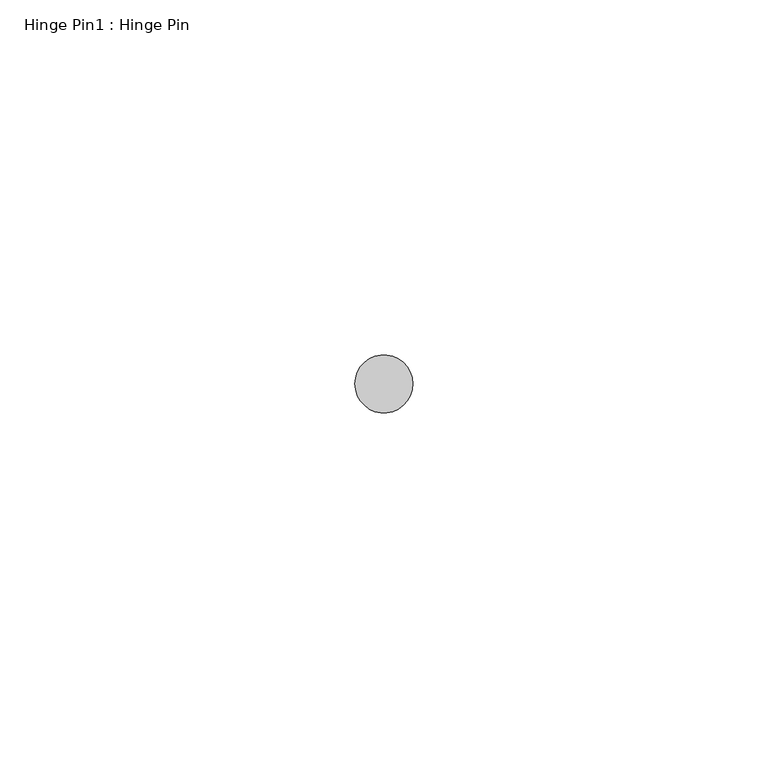
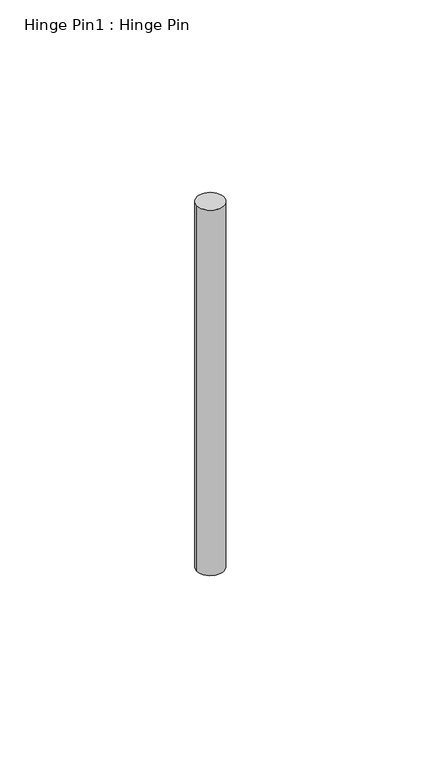
"""IFC4 building model written with IfcOpenShell, lengths in millimetres: proxy geometry, Hinge Pin1 : Hinge Pin."""

from ifc_helpers import new_model, si_unit, point, frame, frame_2d, origin, place, context, project, spatial, circle_curve, trimmed, segment, composite_curve, outline, extrude, source, transform, mapped, element, save


def hinge_pin1_hinge_pin_c6ae77a8(model_context):
    return source(origin(), model_context, "Body", "SweptSolid", [
        extrude(outline(composite_curve([segment(trimmed(circle_curve(frame_2d((587319.1320739, -531776.6049841)), 4.0894), [point((587315.0426739, -531776.6049841))], [point((587323.2214739, -531776.6049841))], False, "CARTESIAN"), True, "CONTINUOUS"), segment(trimmed(circle_curve(frame_2d((587319.1320739, -531776.6049841)), 4.0894), [point((587323.2214739, -531776.6049841))], [point((587315.0426739, -531776.6049841))], False, "CARTESIAN"), True, "CONTINUOUS")], self_intersect=False)), frame((0.0, 0.0, 1941.3140625), z_axis=(0.0, 0.0, 1.0), x_axis=(1.0, 0.0, 0.0)), (0.0, 0.0, 1.0), 117.871875),
    ])


if __name__ == "__main__":
    model = new_model("IFC4")
    model_context = context("Model", 3, world=origin())
    ifc_project = project(units=[si_unit("LENGTHUNIT", "METRE", prefix="MILLI")], contexts=[model_context])
    site = spatial("IfcSite", under=ifc_project)
    building = spatial("IfcBuilding", under=site)
    placement = place(None, origin())
    hinge_pin1_hinge_pin_shape = hinge_pin1_hinge_pin_c6ae77a8(model_context)
    element("IfcBuildingElementProxy", 1, Name="Hinge Pin1 : Hinge Pin", ObjectType="Hinge Pin1 : Hinge Pin", at=placement, inside=building, context=model_context, shape_type="MappedRepresentation", body=[
        mapped(hinge_pin1_hinge_pin_shape, transform((0.0, 0.0, 0.0), x_axis=(1.0, 0.0, 0.0), y_axis=(0.0, 1.0, 0.0), z_axis=(0.0, 0.0, 1.0))),
    ])
    save(model, "model.ifc")

# Revit data of these elements
# Element 1 (IfcBuildingElementProxy, "Hinge Pin1 : Hinge Pin")
#   Materials on its faces: "6\"X6\" WELD-ON STL BUTT HINGE"
# Materials
#   "6\"X6\" WELD-ON STL BUTT HINGE": class "Metal", colour RGB 189 187 185, transparency 0, Description = "Carbon steel", Cost = 0
